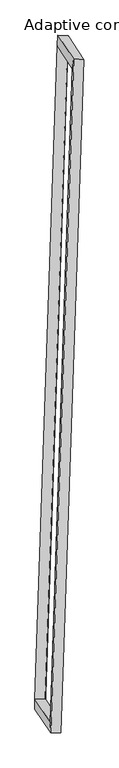
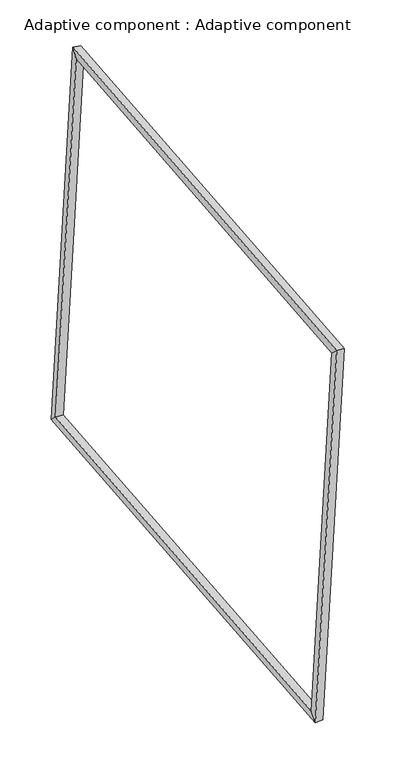
"""IFC4 building model written with IfcOpenShell, lengths in millimetres: proxy geometry, Adaptive component : Adaptive component."""

import ifcopenshell
import ifcopenshell.guid

model = None  # the IFC model being written
_history = None  # IfcOwnerHistory: only IFC2X3 demands one
_inside = {}  # id of a spatial element -> (the spatial element, [elements in it])
_under = {}  # id of a project, library or spatial element -> (it, [spatial elements below it])
_declared = {}  # id of a project -> (the project, [libraries it declares])
_typed = {}  # id of a type object -> (the type object, [elements of that type])
_made_of = {}  # id of a material, layer set ... -> (it, [elements and type objects made of it])


def new_model(schema):
    """Start an empty IFC model of exactly this schema.

    Asked for "IFC4X3", IfcOpenShell would pick the latest addendum, in which some entities
    have other attributes; the version numbers below select the first issue.
    IFC2X3 requires an IfcOwnerHistory on every rooted entity: one is made here for all.
    """
    global model, _history
    if schema == "IFC4X3":
        model = ifcopenshell.file(schema_version=(4, 3, 0, 0))
    else:
        model = ifcopenshell.file(schema=schema)
    _inside.clear()
    _under.clear()
    _declared.clear()
    _typed.clear()
    _made_of.clear()
    _history = None
    if model.schema == "IFC2X3":
        org = make("IfcOrganization", Name="unknown")
        user = make(
            "IfcPersonAndOrganization",
            ThePerson=make("IfcPerson", FamilyName="unknown"),
            TheOrganization=org,
        )
        app = make(
            "IfcApplication",
            ApplicationDeveloper=org,
            Version="unknown",
            ApplicationFullName="unknown",
            ApplicationIdentifier="unknown",
        )
        _history = make(
            "IfcOwnerHistory",
            OwningUser=user,
            OwningApplication=app,
            ChangeAction="ADDED",
            CreationDate=0,
        )
    return model


def make(cls, **values):
    """One entity of the class cls with the attributes given. An attribute that is None is left unset."""
    return model.create_entity(
        cls, **{name: value for name, value in values.items() if value is not None}
    )


def rooted(cls, **values):
    """An entity with a GlobalId (a new one), such as an element, a storey or a relation."""
    return make(cls, GlobalId=ifcopenshell.guid.new(), OwnerHistory=_history, **values)


def si_unit(unit_type, name, prefix=None):
    """IfcSIUnit, for example si_unit("LENGTHUNIT", "METRE", prefix="MILLI")."""
    return make("IfcSIUnit", UnitType=unit_type, Prefix=prefix, Name=name)


def assignment(units):
    """IfcUnitAssignment: the units of a project."""
    return None if units is None else make("IfcUnitAssignment", Units=units)


def point(xyz):
    """IfcCartesianPoint."""
    return None if xyz is None else make("IfcCartesianPoint", Coordinates=xyz)


def direction(xyz):
    """IfcDirection."""
    return None if xyz is None else make("IfcDirection", DirectionRatios=xyz)


def frame(location, z_axis=None, x_axis=None):
    """IfcAxis2Placement3D, a coordinate frame: its origin and axes. An axis left out is left unset."""
    return make(
        "IfcAxis2Placement3D",
        Location=point(location),
        Axis=direction(z_axis),
        RefDirection=direction(x_axis),
    )


def origin():
    """The frame at (0, 0, 0) with its axes left unset."""
    return frame((0.0, 0.0, 0.0))


def place(relative_to, where):
    """IfcLocalPlacement: puts the frame where relative to a parent placement (None: the world)."""
    return make(
        "IfcLocalPlacement", PlacementRelTo=relative_to, RelativePlacement=where
    )


def context(
    kind, dimensions, precision=None, world=None, true_north=None, identifier=None
):
    """IfcGeometricRepresentationContext, for example the 3D "Model" context."""
    return make(
        "IfcGeometricRepresentationContext",
        ContextIdentifier=identifier,
        ContextType=kind,
        CoordinateSpaceDimension=dimensions,
        Precision=precision,
        WorldCoordinateSystem=world,
        TrueNorth=true_north,
    )


def project(units=None, contexts=None):
    """IfcProject with its units and contexts."""
    return rooted(
        "IfcProject",
        Name="project",
        RepresentationContexts=contexts,
        UnitsInContext=assignment(units),
    )


def spatial(cls, under=None, at=None, **own):
    """A site, building, storey or space (cls), placed at a placement, below another one or the project."""
    s = rooted(cls, ObjectPlacement=at, **own)
    if under is not None:
        _under.setdefault(under.id(), (under, []))[1].append(s)
    return s


def faces_of(points, faces, orient=None, outer=None):
    """IfcFace entities. A face is a list of loops; a loop is a list of indices into points, from 0.

    orient and outer hold one flag for each loop. By default every Orientation is true, the
    first loop of a face is its IfcFaceOuterBound and the others are IfcFaceBound.
    """
    made = []
    for i, loops in enumerate(faces):
        bounds = []
        for j, loop in enumerate(loops):
            is_outer = j == 0 if outer is None else outer[i][j]
            bounds.append(
                make(
                    "IfcFaceOuterBound" if is_outer else "IfcFaceBound",
                    Bound=make("IfcPolyLoop", Polygon=[points[k] for k in loop]),
                    Orientation=True if orient is None else orient[i][j],
                )
            )
        made.append(make("IfcFace", Bounds=bounds))
    return made


def faceted_brep(points, faces, orient=None, outer=None, voids=None):
    """IfcFacetedBrep: a solid bounded by flat faces; with voids (closed shells), ...WithVoids."""
    shared = [point(p) for p in points]
    hull = make("IfcClosedShell", CfsFaces=faces_of(shared, faces, orient, outer))
    if voids is None:
        return make("IfcFacetedBrep", Outer=hull)
    return make(
        "IfcFacetedBrepWithVoids",
        Outer=hull,
        Voids=[
            make(cls, CfsFaces=faces_of(shared, fs, o, b)) for cls, fs, o, b in voids
        ],
    )


def shape(context_of_items, identifier, shape_type, items):
    """IfcShapeRepresentation: the items that make up one representation, for example the "Body"."""
    return make(
        "IfcShapeRepresentation",
        ContextOfItems=context_of_items,
        RepresentationIdentifier=identifier,
        RepresentationType=shape_type,
        Items=items,
    )


def source(mapping_origin, context_of_items, identifier, shape_type, items):
    """IfcRepresentationMap: a shape defined once, which mapped items show again and again."""
    return make(
        "IfcRepresentationMap",
        MappingOrigin=mapping_origin,
        MappedRepresentation=shape(context_of_items, identifier, shape_type, items),
    )


def transform(
    local_origin,
    x_axis=None,
    y_axis=None,
    z_axis=None,
    scale=None,
    scale2=None,
    scale3=None,
    uniform=True,
):
    """IfcCartesianTransformationOperator3D, or its non-uniform kind. x_axis, y_axis, z_axis: its Axis1, 2, 3."""
    if uniform:
        return make(
            "IfcCartesianTransformationOperator3D",
            Axis1=direction(x_axis),
            Axis2=direction(y_axis),
            LocalOrigin=point(local_origin),
            Scale=scale,
            Axis3=direction(z_axis),
        )
    return make(
        "IfcCartesianTransformationOperator3DnonUniform",
        Axis1=direction(x_axis),
        Axis2=direction(y_axis),
        LocalOrigin=point(local_origin),
        Scale=scale,
        Axis3=direction(z_axis),
        Scale2=scale2,
        Scale3=scale3,
    )


def mapped(mapping_source, mapping_target):
    """IfcMappedItem: shows the shape of a source again, moved by a transform."""
    return make(
        "IfcMappedItem", MappingSource=mapping_source, MappingTarget=mapping_target
    )


def made_of(thing, what):
    """Note that an element or type object is made of a material, layer set ...; save() writes the relation."""
    if what is not None:
        _made_of.setdefault(what.id(), (what, []))[1].append(thing)
    return thing


def element(
    cls,
    number,
    at=None,
    inside=None,
    cuts=None,
    type_object=None,
    material=None,
    context=None,
    identifier="Body",
    shape_type=None,
    held_by="IfcProductDefinitionShape",
    body=None,
    shapes=None,
    **own,
):
    """One element of the class cls, such as IfcWall. Its Tag is "e" and its number.

    at: its placement. inside: the storey or other place that contains it. cuts: it is an
    opening in that element (IfcRelVoidsElement). A single representation is given by context,
    identifier, shape_type and body (its items); several are given by shapes. held_by: the class
    of the entity that holds the representations. save() writes the other relations.
    """
    e = rooted(cls, Tag="e%d" % number, ObjectPlacement=at, **own)
    if body is not None:
        shapes = [shape(context, identifier, shape_type, body)]
    if shapes is not None:
        e.Representation = make(held_by, Representations=shapes)
    if inside is not None:
        _inside.setdefault(inside.id(), (inside, []))[1].append(e)
    if cuts is not None:
        rooted(
            "IfcRelVoidsElement", RelatingBuildingElement=cuts, RelatedOpeningElement=e
        )
    if type_object is not None:
        _typed.setdefault(type_object.id(), (type_object, []))[1].append(e)
    return made_of(e, material)


def aggregate(whole, parts):
    """IfcRelAggregates: a whole, such as a stair, and the parts it consists of."""
    return rooted("IfcRelAggregates", RelatingObject=whole, RelatedObjects=parts)


def save(model, path):
    """Write the relations noted so far, then the file.

    IfcRelAggregates (storeys below a building ...), IfcRelContainedInSpatialStructure (elements
    in a storey), IfcRelDefinesByType, IfcRelAssociatesMaterial and IfcRelDeclares: one each for
    every whole, place, type object, material and project.
    """
    for whole, parts in _under.values():
        aggregate(whole, parts)
    for where, things in _inside.values():
        rooted(
            "IfcRelContainedInSpatialStructure",
            RelatedElements=things,
            RelatingStructure=where,
        )
    for kind, things in _typed.values():
        rooted("IfcRelDefinesByType", RelatedObjects=things, RelatingType=kind)
    for what, things in _made_of.values():
        rooted("IfcRelAssociatesMaterial", RelatedObjects=things, RelatingMaterial=what)
    for by, libraries in _declared.values():
        rooted("IfcRelDeclares", RelatingContext=by, RelatedDefinitions=libraries)
    model.write(path)


def adaptive_component_adaptive_component_2d6e63bc(model_context):
    return source(origin(), model_context, "Body", "Brep", [
        faceted_brep([(94.4993372, 1567.583495, 3118.5221644), (159.1075647, 1561.9900346, 3112.8090425), (18.8026024, -2550.4923425, 2938.3361202), (-46.0526911, -2552.1406412, 2943.742009), (102.1779266, 1629.454713, 3185.9746812), (-42.7958376, -2619.8750394, 3005.6959805), (166.7861541, 1623.8612526, 3180.2615593), (22.0594559, -2618.2267407, 3000.2900917), (-76.9158177, -2404.5794904, -423.9865595), (-141.9772971, -2405.9134802, -425.8234054), (-142.4105463, -2468.0226976, -493.4925104), (-77.3490669, -2466.6887078, -491.6556646), (63.3891446, 1707.9028867, -249.5136372), (-1.4252687, 1713.8106561, -251.04325), (2.563218, 1781.3070548, -313.2138097), (67.3776313, 1775.3992855, -311.684197)], [[[0, 1, 2, 3]], [[4, 0, 3, 5]], [[6, 4, 5, 7]], [[1, 6, 7, 2]], [[3, 2, 8, 9]], [[5, 3, 9, 10]], [[7, 5, 10, 11]], [[2, 7, 11, 8]], [[9, 8, 12, 13]], [[10, 9, 13, 14]], [[11, 10, 14, 15]], [[8, 11, 15, 12]], [[13, 12, 1, 0]], [[14, 13, 0, 4]], [[15, 14, 4, 6]], [[12, 15, 6, 1]]]),
    ])


if __name__ == "__main__":
    model = new_model("IFC4")
    model_context = context("Model", 3, world=origin())
    ifc_project = project(units=[si_unit("LENGTHUNIT", "METRE", prefix="MILLI")], contexts=[model_context])
    site = spatial("IfcSite", under=ifc_project)
    building = spatial("IfcBuilding", under=site)
    placement = place(None, origin())
    adaptive_component_adaptive_component_shape = adaptive_component_adaptive_component_2d6e63bc(model_context)
    element("IfcBuildingElementProxy", 1, Name="Adaptive component : Adaptive component", ObjectType="Adaptive component : Adaptive component", at=placement, inside=building, context=model_context, shape_type="MappedRepresentation", body=[
        mapped(adaptive_component_adaptive_component_shape, transform((0.0, 0.0, 0.0), x_axis=(1.0, 0.0, 0.0), y_axis=(0.0, 1.0, 0.0), z_axis=(0.0, 0.0, 1.0))),
    ])
    save(model, "model.ifc")

# Revit data of these elements
# Type "Adaptive component : Adaptive component"
#   r [instance default] = 2063.125 mm
#   2r [instance default] = 4126.251 mm
#   Number [instance default] = 5
#   Default Elevation = 0
# Element 1 (IfcBuildingElementProxy, "Adaptive component : Adaptive component")
#   r = 2753.505 mm
#   2r = 5507.01 mm
#   Number = 29
